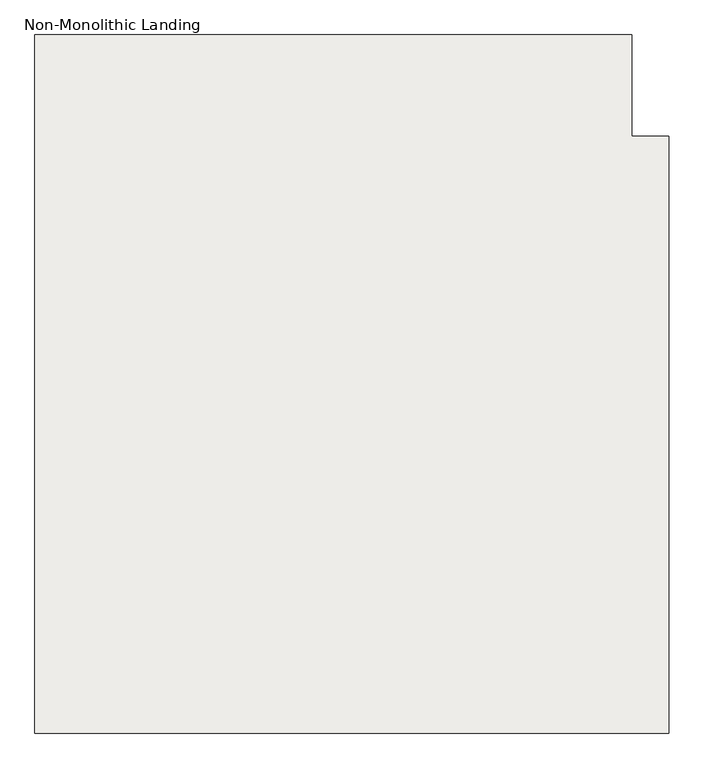
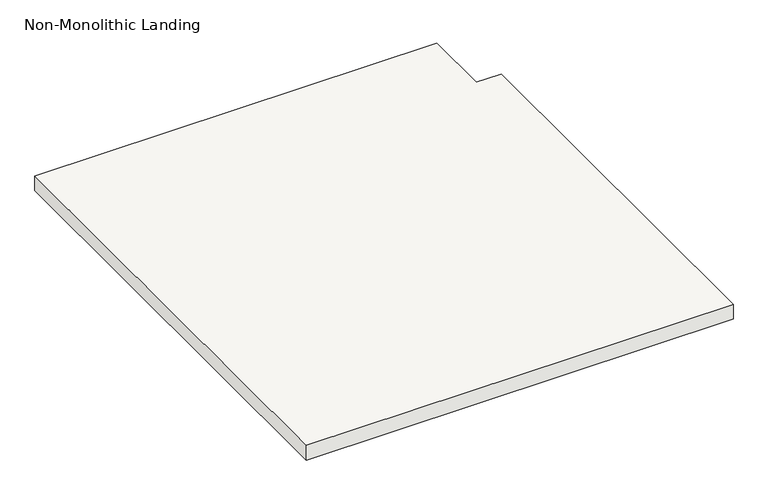
"""IFC4 building model written with IfcOpenShell, lengths in millimetres: slab geometry, Non-Monolithic Landing."""

from ifc_helpers import new_model, si_unit, frame, origin, place, context, project, spatial, polyline, outline, extrude, source, transform, mapped, element, save


def non_monolithic_landing_61911332(model_context):
    return source(origin(), model_context, "Body", "SweptSolid", [
        extrude(outline(polyline([(-13195.5859635, -3119.3642494), (-14576.101437, -3119.3642494), (-14576.101437, -1598.3427081), (-13276.101437, -1598.3427081), (-13276.101437, -1819.3642494), (-13195.5859635, -1819.3642494), (-13195.5859635, -3119.3642494)])), frame((0.0, 0.0, 4270.0), z_axis=(0.0, 0.0, 1.0), x_axis=(1.0, 0.0, 0.0)), (0.0, 0.0, 1.0), 50.0),
    ])


if __name__ == "__main__":
    model = new_model("IFC4")
    model_context = context("Model", 3, world=origin())
    ifc_project = project(units=[si_unit("LENGTHUNIT", "METRE", prefix="MILLI")], contexts=[model_context])
    site = spatial("IfcSite", under=ifc_project)
    building = spatial("IfcBuilding", under=site)
    placement = place(None, origin())
    non_monolithic_landing_shape = non_monolithic_landing_61911332(model_context)
    element("IfcSlab", 1, ObjectType="Non-Monolithic Landing", at=placement, inside=building, context=model_context, shape_type="MappedRepresentation", body=[
        mapped(non_monolithic_landing_shape, transform((0.0, 0.0, 0.0), x_axis=(1.0, 0.0, 0.0), y_axis=(0.0, 1.0, 0.0), z_axis=(0.0, 0.0, 1.0))),
    ])
    save(model, "model.ifc")
